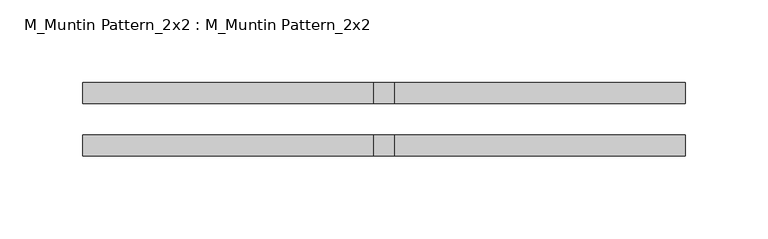
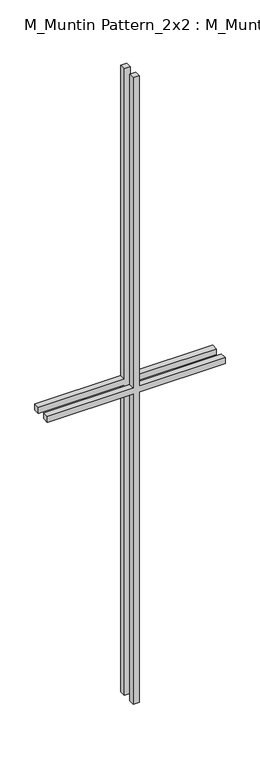
"""IFC4 building model written with IfcOpenShell, lengths in millimetres: proxy geometry, M_Muntin Pattern_2x2 : M_Muntin Pattern_2x2."""

from ifc_helpers import new_model, si_unit, frame, origin, place, context, project, spatial, polyline, outline, extrude, source, transform, mapped, element, save


def m_muntin_pattern_2x2_m_muntin_pattern_2x2_b334ec9d(model_context):
    return source(origin(), model_context, "Body", "SweptSolid", [
        extrude(outline(polyline([(686.5, -6.35), (686.5, -182.2666667), (673.8, -182.2666667), (673.8, -6.35), (0.0, -6.35), (0.0, 6.35), (673.8, 6.35), (673.8, 182.2666667), (686.5, 182.2666667), (686.5, 6.35), (1360.3, 6.35), (1360.3, -6.35), (686.5, -6.35)])), frame((0.0, 9.525, 0.0), z_axis=(0.0, 1.0, 0.0), x_axis=(0.0, 0.0, 1.0)), (0.0, 0.0, 1.0), 12.7),
        extrude(outline(polyline([(686.5, -6.35), (686.5, -182.2666667), (673.8, -182.2666667), (673.8, -6.35), (0.0, -6.35), (0.0, 6.35), (673.8, 6.35), (673.8, 182.2666667), (686.5, 182.2666667), (686.5, 6.35), (1360.3, 6.35), (1360.3, -6.35), (686.5, -6.35)])), frame((0.0, -22.225, 0.0), z_axis=(0.0, 1.0, 0.0), x_axis=(0.0, 0.0, 1.0)), (0.0, 0.0, 1.0), 12.7),
    ])


if __name__ == "__main__":
    model = new_model("IFC4")
    model_context = context("Model", 3, world=origin())
    ifc_project = project(units=[si_unit("LENGTHUNIT", "METRE", prefix="MILLI")], contexts=[model_context])
    site = spatial("IfcSite", under=ifc_project)
    building = spatial("IfcBuilding", under=site)
    placement = place(None, origin())
    m_muntin_pattern_2x2_m_muntin_pattern_2x2_shape = m_muntin_pattern_2x2_m_muntin_pattern_2x2_b334ec9d(model_context)
    element("IfcBuildingElementProxy", 1, Name="M_Muntin Pattern_2x2 : M_Muntin Pattern_2x2", ObjectType="M_Muntin Pattern_2x2 : M_Muntin Pattern_2x2", at=placement, inside=building, context=model_context, shape_type="MappedRepresentation", body=[
        mapped(m_muntin_pattern_2x2_m_muntin_pattern_2x2_shape, transform((0.0, 0.0, 0.0), x_axis=(1.0, 0.0, 0.0), y_axis=(0.0, 1.0, 0.0), z_axis=(0.0, 0.0, 1.0))),
    ])
    save(model, "model.ifc")

# Revit data of these elements
# Type "M_Muntin Pattern_2x2 : M_Muntin Pattern_2x2"
#   Width [instance default] = 1.2 m
#   Thickness = 0.0127 m
#   Height [instance default] = 1.2 m
#   Distance = 0.01905 m
#   Interior Material [instance default] = none
#   Exterior Material [instance default] = none
# Element 1 (IfcBuildingElementProxy, "M_Muntin Pattern_2x2 : M_Muntin Pattern_2x2")
#   Width = 0.364533 m
#   Height = 1.3603 m
#   Interior Material = Wood - Stained
#   Exterior Material = Clad - White
#   Materials on its faces: "Clad - White", "Wood - Stained"
# Materials
#   "Clad - White": class "Wood", colour RGB 242 242 238, transparency 0, Cost = 0
#   "Wood - Stained": class "Wood", colour RGB 224 178 126, transparency 0, Cost = 0
